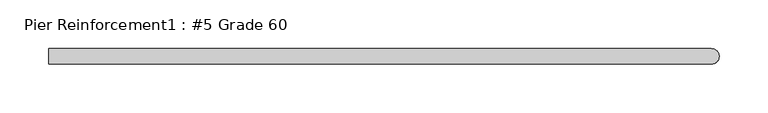
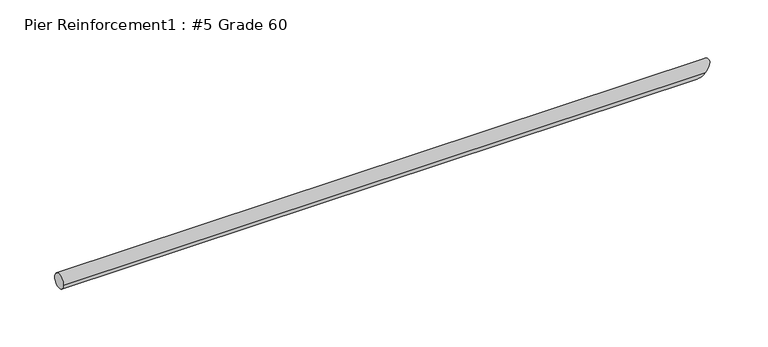
"""IFC4 building model written with IfcOpenShell, lengths in millimetres: proxy geometry, Pier Reinforcement1 : #5 Grade 60."""

from ifc_helpers import new_model, si_unit, frame, origin, place, context, project, spatial, circle_curve, ellipse_curve, source, transform, mapped, element, save
from ifc_brep_helpers import plane_surface, cylinder_surface, advanced_brep


def pier_reinforcement1_5_grade_60_09892ae6(model_context):
    return source(origin(), model_context, "Body", "AdvancedBrep", [
        advanced_brep(
        [(589548.1922365, -534037.9288841, -55.5625), (589548.1922365, -534053.8038841, -55.5625), (590226.0547365, -534053.8038841, -55.5625), (590233.9922365, -534045.8663841, -47.625), (590226.0547365, -534037.9288841, -55.5625), (590218.1172365, -534045.8663841, -63.5)],
        [
            (0, 1, circle_curve(frame((589548.1922365, -534045.8663841, -55.5625), z_axis=(-1.0, 0.0, 0.0), x_axis=(0.0, -1.0, 0.0)), 7.9375)),
            (1, 0, circle_curve(frame((589548.1922365, -534045.8663841, -55.5625), z_axis=(-1.0, 0.0, 0.0), x_axis=(0.0, -1.0, 0.0)), 7.9375)),
            (1, 2),
            (2, 3, ellipse_curve(frame((590226.0547365, -534045.8663841, -55.5625), z_axis=(-0.7071067811865462, 0.0, 0.7071067811865489), x_axis=(0.7071067811865487, 0.0, 0.7071067811865462)), 11.2253202, 7.9375)),
            (3, 4, ellipse_curve(frame((590226.0547365, -534045.8663841, -55.5625), z_axis=(-0.7071067811865462, 0.0, 0.7071067811865489), x_axis=(0.7071067811865487, 0.0, 0.7071067811865462)), 11.2253202, 7.9375)),
            (4, 0),
            (4, 5, ellipse_curve(frame((590226.0547365, -534045.8663841, -55.5625), z_axis=(-0.7071067811865462, 0.0, 0.7071067811865489), x_axis=(0.7071067811865487, 0.0, 0.7071067811865462)), 11.2253202, 7.9375)),
            (5, 2, ellipse_curve(frame((590226.0547365, -534045.8663841, -55.5625), z_axis=(-0.7071067811865462, 0.0, 0.7071067811865489), x_axis=(0.7071067811865487, 0.0, 0.7071067811865462)), 11.2253202, 7.9375)),
        ],
        [
            plane_surface(frame((589548.1922365, -534053.8038841, -55.5625), z_axis=(-1.0, 0.0, 0.0), x_axis=(0.0, 0.0, 1.0))),
            cylinder_surface(frame((589548.1922365, -534045.8663841, -55.5625), z_axis=(1.0, 0.0, 0.0), x_axis=(0.0, -1.0, 0.0)), 7.9375),
            plane_surface(frame((590218.1172365, -534020.4663841, -63.5), z_axis=(0.7071067811865462, 0.0, -0.7071067811865489), x_axis=(0.0, -1.0, 0.0))),
        ],
        [
            (0, [[1, 2]]),
            (1, [[-2, 3, 4, 5, 6]]),
            (1, [[-1, -6, 7, 8, -3]]),
            (2, [[-5, -4, -8, -7]]),
        ],
    ),
    ])


if __name__ == "__main__":
    model = new_model("IFC4")
    model_context = context("Model", 3, world=origin())
    ifc_project = project(units=[si_unit("LENGTHUNIT", "METRE", prefix="MILLI")], contexts=[model_context])
    site = spatial("IfcSite", under=ifc_project)
    building = spatial("IfcBuilding", under=site)
    placement = place(None, origin())
    pier_reinforcement1_5_grade_60_shape = pier_reinforcement1_5_grade_60_09892ae6(model_context)
    element("IfcBuildingElementProxy", 1, Name="Pier Reinforcement1 : #5 Grade 60", ObjectType="Pier Reinforcement1 : #5 Grade 60", at=placement, inside=building, context=model_context, shape_type="MappedRepresentation", body=[
        mapped(pier_reinforcement1_5_grade_60_shape, transform((0.0, 0.0, 0.0), x_axis=(1.0, 0.0, 0.0), y_axis=(0.0, 1.0, 0.0), z_axis=(0.0, 0.0, 1.0))),
    ])
    save(model, "model.ifc")

# Revit data of these elements
# Element 1 (IfcBuildingElementProxy, "Pier Reinforcement1 : #5 Grade 60")
#   Materials on its faces: "#5 GR. 60 BEND 24\"x24\""
# Materials
#   "#5 GR. 60 BEND 24\"x24\"": class "Generic", colour RGB 84 83 81, transparency 0, Cost = 0
